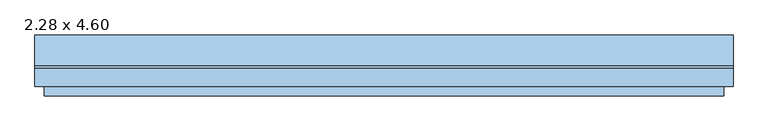
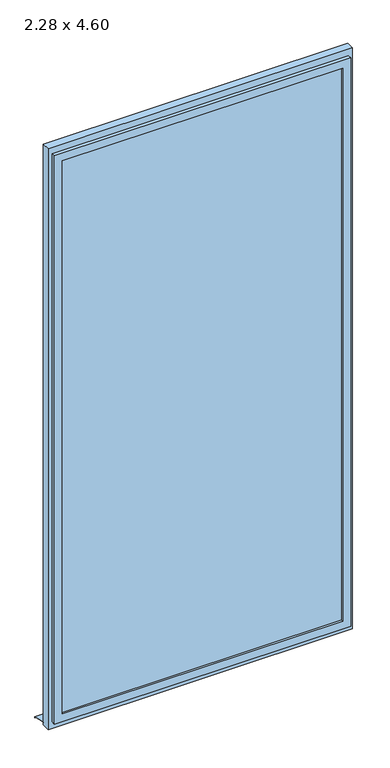
"""IFC4 building model written with IfcOpenShell, lengths in millimetres: window geometry, Fenstertür 1-flg : 2.28 x 4.60."""

from ifc_helpers import new_model, si_unit, frame, origin, place, context, project, spatial, polyline, outline, extrude, faceted_brep, source, transform, mapped, element, save


def window_2_28_x_4_60_34926950(model_context):
    return source(origin(), model_context, "Body", "SolidModel", [
        extrude(outline(polyline([(4600.0, 1140.0), (4600.0, -1140.0), (0.0, -1140.0), (0.0, 1140.0), (4600.0, 1140.0)]), holes=[polyline([(4520.0, 1080.0), (80.0, 1080.0), (80.0, -1080.0), (4520.0, -1080.0), (4520.0, 1080.0)])]), frame((0.0, -80.0, 0.0), z_axis=(0.0, 1.0, 0.0), x_axis=(0.0, 0.0, 1.0)), (0.0, 0.0, 1.0), 60.0),
        faceted_brep([(1110.0, -80.0, 4550.0), (1110.0, -110.0, 4550.0), (1110.0, -110.0, 50.0), (1110.0, -80.0, 50.0), (-1110.0, -110.0, 4550.0), (-1110.0, -110.0, 50.0), (1050.0, -110.0, 110.0), (-1050.0, -110.0, 110.0), (-1050.0, -110.0, 4490.0), (1050.0, -110.0, 4490.0), (-1110.0, -80.0, 50.0), (-1110.0, -80.0, 4550.0), (1080.0, -80.0, 4520.0), (-1080.0, -80.0, 4520.0), (-1080.0, -80.0, 80.0), (1080.0, -80.0, 80.0), (1080.0, -50.0, 4520.0), (1080.0, -50.0, 80.0), (-1080.0, -50.0, 80.0), (-1080.0, -50.0, 4520.0), (1050.0, -50.0, 4490.0), (-1050.0, -50.0, 4490.0), (-1050.0, -50.0, 110.0), (1050.0, -50.0, 110.0)], [[[0, 1, 2, 3]], [[1, 4, 5, 2], [6, 7, 8, 9]], [[3, 2, 5, 10]], [[3, 10, 11, 0], [12, 13, 14, 15]], [[16, 12, 15, 17]], [[17, 15, 14, 18]], [[17, 18, 19, 16], [20, 21, 22, 23]], [[9, 20, 23, 6]], [[6, 23, 22, 7]], [[10, 5, 4, 11]], [[18, 14, 13, 19]], [[7, 22, 21, 8]], [[11, 4, 1, 0]], [[19, 13, 12, 16]], [[8, 21, 20, 9]]]),
        extrude(outline(polyline([(-9.9778457, 20.0), (90.0, 0.0), (90.0, -10.0), (88.0, -10.0), (88.0, -1.6395366), (-10.1759277, 18.0), (-20.0, 18.0), (-20.0, 20.0), (-9.9778457, 20.0)])), frame((-1140.0, 0.0, 0.0), z_axis=(1.0, 0.0, 0.0), x_axis=(0.0, 1.0, 0.0)), (0.0, 0.0, 1.0), 2280.0),
        extrude(outline(polyline([(1050.0, -95.0), (-1050.0, -95.0), (-1050.0, -65.0), (1050.0, -65.0), (1050.0, -95.0)])), frame((0.0, 0.0, 110.0), z_axis=(0.0, 0.0, 1.0), x_axis=(1.0, 0.0, 0.0)), (0.0, 0.0, 1.0), 4380.0),
    ])


if __name__ == "__main__":
    model = new_model("IFC4")
    model_context = context("Model", 3, world=origin())
    ifc_project = project(units=[si_unit("LENGTHUNIT", "METRE", prefix="MILLI")], contexts=[model_context])
    site = spatial("IfcSite", under=ifc_project)
    building = spatial("IfcBuilding", under=site)
    placement = place(None, origin())
    window_2_28_x_4_60_shape = window_2_28_x_4_60_34926950(model_context)
    element("IfcWindow", 1, ObjectType="Fenstertür 1-flg : 2.28 x 4.60", at=placement, inside=building, context=model_context, shape_type="MappedRepresentation", body=[
        mapped(window_2_28_x_4_60_shape, transform((0.0, 0.0, 0.0), x_axis=(1.0, 0.0, 0.0), y_axis=(0.0, 1.0, 0.0), z_axis=(0.0, 0.0, 1.0))),
    ])
    save(model, "model.ifc")

# Revit data of these elements
# Type "Fenstertür 1-flg : 2.28 x 4.60"
#   Type Mark = "60"
#   Operation = "SinglePanel"
#   Construction Type Id = "SGL"
#   Keynote = "16.05.01"
#   Analytic Construction = "Große Fenster mit Einfachverglasung"
#   Visual Light Transmittance = 0.9
#   Solar Heat Gain Coefficient = 0.86
#   Rough Width = 2.280 m
#   Rough Height = 4.600 m
#   Heat Transfer Coefficient (U) = 5.5617 W/(m²·K)
#   Rahmentiefe = 0.060 m
#   Rahmenhöhe unten = 0.080 m
#   Höhe oberer  Rahmen = 0.080 m
#   Rahmenbreite = 0.060 m
#   Height = 4.600 m
#   Tiefe Flügel = 0.060 m
#   Flügelbreite = 0.060 m
#   Einbautiefe (von außen) [instance default] = 0.080 m
#   Width = 2.280 m
#   Sichtbarkeit Sturzlinien [instance default] = yes
#   Öffnungsrichtung oben [instance default] = yes
#   Öffnungsrichtung in Draufsicht anzeigen [instance default] = yes
#   Drehflügel 1 [instance default] = yes
#   Bild [instance default] = none
#   Glas [instance default] = none
#   Fensterflügel [instance default] = none
#   Äußere Fensterbank [instance default] = none
#   Wall Closure = (empty or 0)
# Element 1 (IfcWindow, "Fenstertür 1-flg : 2.28 x 4.60")
#   Materials on its faces: "Kunststoff - Weiß", "Glas"
# Materials
#   "Kunststoff - Weiß": class "Kunststoff", colour RGB 249 249 249, transparency 0, Cost = 0
#   "Glas": class "Glas", colour RGB 0 0 255, transparency 0.75, Comments = "Render-Darstellung nicht aktualisiert ", Cost = 0
